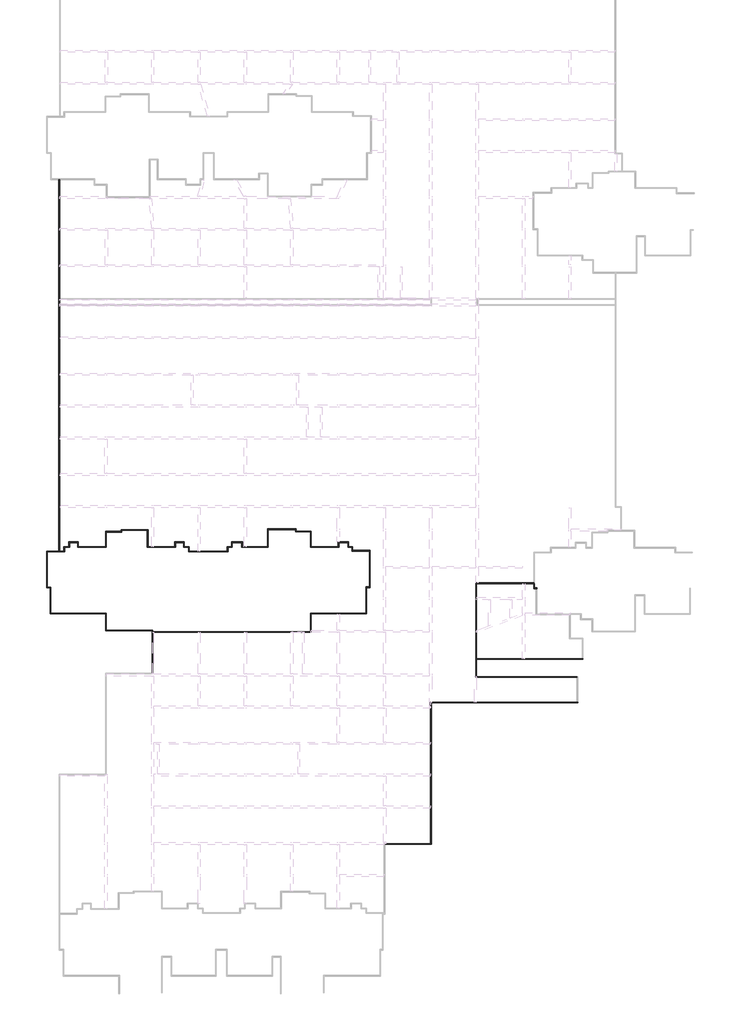
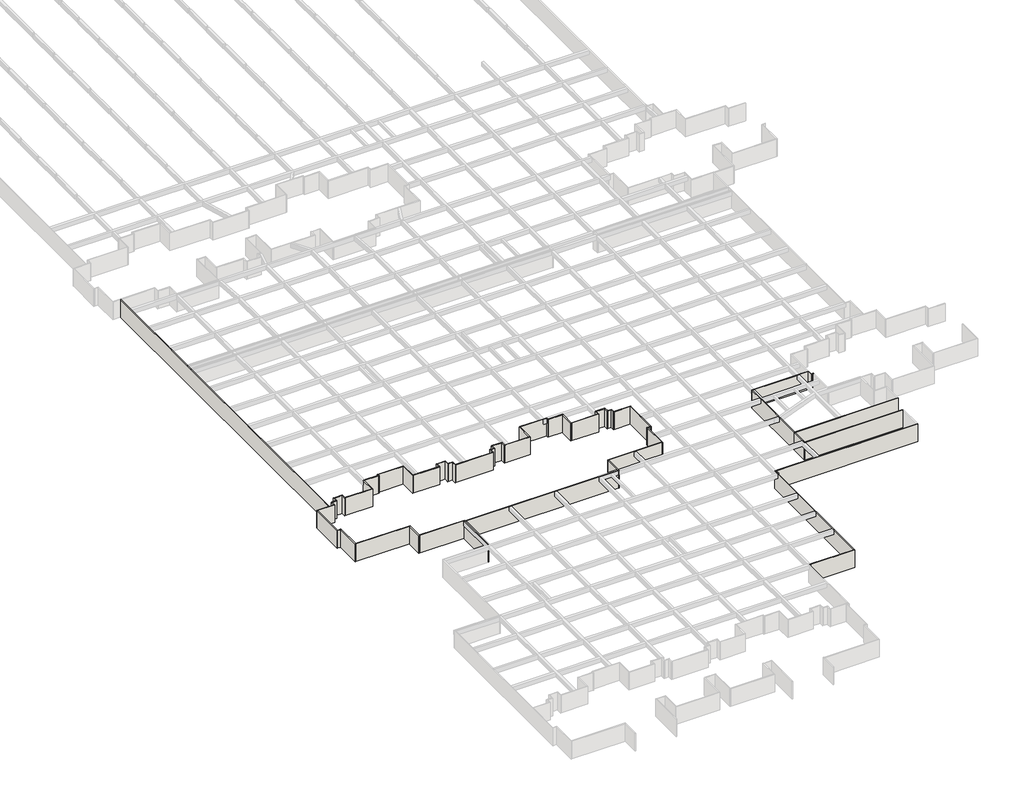
# One storey, part 2 of 14: 61 walls.
"""IFC4 building model written with IfcOpenShell, lengths in millimetres."""

from ifc_helpers import new_model, si_unit, origin, origin_with_axes, place, context, project, spatial, polyline, outline, extrude, faceted_brep, element, save

model = new_model("IFC4")

# Units and contexts
model_context = context("Model", 3, world=origin())
ifc_project = project(units=[si_unit("LENGTHUNIT", "METRE", prefix="MILLI")], contexts=[model_context])

# Site, building, storey
site = spatial("IfcSite", under=ifc_project)
building = spatial("IfcBuilding", under=site)
storey = spatial("IfcBuildingStorey", under=building, Name="户型图", Elevation=0.0)

# Walls
placement = place(None, origin())
element("IfcWall", 1, ObjectType="所有墙体", at=placement, inside=storey, context=model_context, shape_type="Brep", body=[
    faceted_brep([(-594257.5937933, -107575.8355437, 0.0), (-594257.5937933, -171682.856538, 0.0), (-594257.5937933, -171682.856538, 3300.0), (-594257.5937933, -107575.8355437, 3300.0), (-594137.5937933, -107575.8355437, 0.0), (-594137.5937933, -107575.8355437, 3300.0), (-594137.5937933, -128099.4327532, 3300.0), (-594137.5937933, -128219.4327532, 3300.0), (-594137.5937933, -129174.4327531, 3300.0), (-594137.5937933, -129294.4327531, 3300.0), (-594137.5937933, -171682.856538, 3300.0), (-594137.5937933, -171682.856538, 0.0), (-594137.5937933, -129294.4327531, 0.0), (-594137.5937933, -129174.4327531, 0.0), (-594137.5937933, -128219.4327532, 0.0), (-594137.5937933, -128099.4327532, 0.0)], [[[0, 1, 2, 3]], [[4, 5, 6, 7, 8, 9, 10, 11, 12, 13, 14, 15]], [[1, 0, 4, 15, 14, 13, 12, 11]], [[3, 2, 10, 9, 8, 7, 6, 5]], [[0, 3, 5, 4]], [[2, 1, 11, 10]]]),
])
element("IfcWall", 2, ObjectType="所有墙体", at=placement, inside=storey, context=model_context, shape_type="Brep", body=[
    faceted_brep([(-593271.2602583, -171682.856538, 0.0), (-593391.2602583, -171682.856538, 0.0), (-594137.5937933, -171682.856538, 0.0), (-594257.5937933, -171682.856538, 0.0), (-596391.260259, -171682.856538, 0.0), (-596391.260259, -171682.856538, 3300.0), (-594257.5937933, -171682.856538, 3300.0), (-594137.5937933, -171682.856538, 3300.0), (-593391.2602583, -171682.856538, 3300.0), (-593271.2602583, -171682.856538, 3300.0), (-593271.2602583, -171802.856538, 0.0), (-593271.2602583, -171802.856538, 3300.0), (-596271.260259, -171802.856538, 3300.0), (-596391.260259, -171802.856538, 3300.0), (-596391.260259, -171802.856538, 0.0), (-596271.260259, -171802.856538, 0.0)], [[[0, 1, 2, 3, 4, 5, 6, 7, 8, 9]], [[10, 11, 12, 13, 14, 15]], [[4, 3, 2, 1, 0, 10, 15, 14]], [[9, 8, 7, 6, 5, 13, 12, 11]], [[5, 4, 14, 13]], [[0, 9, 11, 10]]]),
])
element("IfcWall", 3, ObjectType="所有墙体", at=placement, inside=storey, context=model_context, shape_type="Brep", body=[
    faceted_brep([(-596391.260259, -171802.856538, 0.0), (-596391.260259, -178002.8565379, 0.0), (-596391.260259, -178002.8565379, 3300.0), (-596391.260259, -171802.856538, 3300.0), (-596271.260259, -171802.856538, 0.0), (-596271.260259, -171802.856538, 3300.0), (-596271.260259, -177882.8565379, 3300.0), (-596271.260259, -178002.8565379, 3300.0), (-596271.260259, -178002.8565379, 0.0), (-596271.260259, -177882.8565379, 0.0)], [[[0, 1, 2, 3]], [[4, 5, 6, 7, 8, 9]], [[1, 0, 4, 9, 8]], [[3, 2, 7, 6, 5]], [[0, 3, 5, 4]], [[2, 1, 8, 7]]]),
])
element("IfcWall", 4, ObjectType="所有墙体", at=placement, inside=storey, context=model_context, shape_type="Brep", body=[
    faceted_brep([(-596271.260259, -178002.8565379, 0.0), (-595791.2602578, -178002.8565379, 0.0), (-595671.2602578, -178002.8565379, 0.0), (-595671.2602578, -178002.8565379, 3300.0), (-595791.2602578, -178002.8565379, 3300.0), (-596271.260259, -178002.8565379, 3300.0), (-596271.260259, -177882.8565379, 0.0), (-596271.260259, -177882.8565379, 3300.0), (-595671.2602578, -177882.8565379, 3300.0), (-595671.2602578, -177882.8565379, 0.0)], [[[0, 1, 2, 3, 4, 5]], [[6, 7, 8, 9]], [[2, 1, 0, 6, 9]], [[5, 4, 3, 8, 7]], [[0, 5, 7, 6]], [[3, 2, 9, 8]]]),
])
element("IfcWall", 5, ObjectType="所有墙体", at=placement, inside=storey, context=model_context, shape_type="Brep", body=[
    faceted_brep([(-595791.2602578, -178002.8565379, 0.0), (-595791.2602578, -182502.856538, 0.0), (-595791.2602578, -182502.856538, 3300.0), (-595791.2602578, -178002.8565379, 3300.0), (-595671.2602578, -178002.8565379, 0.0), (-595671.2602578, -178002.8565379, 3300.0), (-595671.2602578, -182382.856538, 3300.0), (-595671.2602578, -182502.856538, 3300.0), (-595671.2602578, -182502.856538, 0.0), (-595671.2602578, -182382.856538, 0.0)], [[[0, 1, 2, 3]], [[4, 5, 6, 7, 8, 9]], [[1, 0, 4, 9, 8]], [[3, 2, 7, 6, 5]], [[0, 3, 5, 4]], [[2, 1, 8, 7]]]),
])
element("IfcWall", 6, ObjectType="所有墙体", at=placement, inside=storey, context=model_context, shape_type="Brep", body=[
    faceted_brep([(-595671.2602578, -182502.856538, 0.0), (-586191.2602569, -182502.856538, 0.0), (-586071.2602569, -182502.856538, 0.0), (-586071.2602569, -182502.856538, 3300.0), (-586191.2602569, -182502.856538, 3300.0), (-595671.2602578, -182502.856538, 3300.0), (-595671.2602578, -182382.856538, 0.0), (-595671.2602578, -182382.856538, 3300.0), (-586071.2602569, -182382.856538, 3300.0), (-586071.2602569, -182382.856538, 0.0)], [[[0, 1, 2, 3, 4, 5]], [[6, 7, 8, 9]], [[2, 1, 0, 6, 9]], [[5, 4, 3, 8, 7]], [[0, 5, 7, 6]], [[3, 2, 9, 8]]]),
])
element("IfcWall", 7, ObjectType="所有墙体", at=placement, inside=storey, context=model_context, shape_type="Brep", body=[
    faceted_brep([(-586191.2602569, -182502.856538, 0.0), (-586191.2602569, -185431.2417661, 0.0), (-586191.2602569, -185431.2417661, 3300.0), (-586191.2602569, -182502.856538, 3300.0), (-586071.2602569, -182502.856538, 0.0), (-586071.2602569, -182502.856538, 3300.0), (-586071.2602569, -185311.2417661, 3300.0), (-586071.2602569, -185431.2417661, 3300.0), (-586071.2602569, -185431.2417661, 0.0), (-586071.2602569, -185311.2417661, 0.0)], [[[0, 1, 2, 3]], [[4, 5, 6, 7, 8, 9]], [[1, 0, 4, 9, 8]], [[3, 2, 7, 6, 5]], [[0, 3, 5, 4]], [[2, 1, 8, 7]]]),
])
element("IfcWall", 8, ObjectType="所有墙体", at=placement, inside=storey, context=model_context, shape_type="Brep", body=[
    faceted_brep([(-586071.2602569, -185431.2417661, 0.0), (-578191.2602569, -185431.2417661, 0.0), (-578071.2602569, -185431.2417661, 0.0), (-578071.2602569, -185431.2417661, 3300.0), (-578191.2602569, -185431.2417661, 3300.0), (-578267.6529954, -185431.2417661, 3300.0), (-586071.2602569, -185431.2417661, 3300.0), (-586071.2602569, -185311.2417661, 0.0), (-586071.2602569, -185311.2417661, 3300.0), (-578071.2602569, -185311.2417661, 3300.0), (-578071.2602569, -185311.2417661, 0.0), (-578071.2602569, -185371.5491398, 3300.0)], [[[0, 1, 2, 3, 4, 5, 6]], [[7, 8, 9, 10]], [[2, 1, 0, 7, 10]], [[6, 5, 4, 3, 11, 9, 8]], [[0, 6, 8, 7]], [[3, 2, 10, 9, 11]]]),
])
element("IfcWall", 9, ObjectType="所有墙体", at=placement, inside=storey, context=model_context, shape_type="Brep", body=[
    faceted_brep([(-578191.2602569, -185431.2417661, 0.0), (-578191.2602569, -192711.2417661, 0.0), (-578191.2602569, -192831.2417661, 0.0), (-578191.2602569, -192831.2417661, 3300.0), (-578191.2602569, -192711.2417661, 3300.0), (-578191.2602569, -185431.2417661, 3300.0), (-578191.2602569, -185431.2417661, 2500.0), (-578071.2602569, -185431.2417661, 0.0), (-578071.2602569, -185431.2417661, 3300.0), (-578071.2602569, -185532.8564588, 3300.0), (-578071.2602569, -185652.8564588, 3300.0), (-578071.2602569, -192831.2417661, 3300.0), (-578071.2602569, -192831.2417661, 2500.0), (-578071.2602569, -192831.2417661, 0.0), (-578071.2602569, -185652.8564588, 0.0), (-578071.2602569, -185532.8564588, 0.0)], [[[0, 1, 2, 3, 4, 5, 6]], [[7, 8, 9, 10, 11, 12, 13, 14, 15]], [[2, 1, 0, 7, 15, 14, 13]], [[5, 4, 3, 11, 10, 9, 8]], [[0, 6, 5, 8, 7]], [[3, 2, 13, 12, 11]]]),
])
element("IfcWall", 10, ObjectType="所有墙体", at=placement, inside=storey, context=model_context, shape_type="Brep", body=[
    faceted_brep([(-537997.7352575, -222250.9174567, 0.0), (-529997.7352575, -222250.9174567, 0.0), (-529997.7352575, -222250.9174567, 3300.0), (-537831.2602569, -222250.9174567, 3300.0), (-537997.7352575, -222250.9174567, 3300.0), (-537997.7352575, -222250.9174567, 2500.0), (-537997.7352575, -222130.9174567, 0.0), (-537997.7352575, -222130.9174567, 3300.0), (-537831.2602569, -222130.9174567, 3300.0), (-530117.7352575, -222130.9174567, 3300.0), (-529997.7352575, -222130.9174567, 3300.0), (-529997.7352575, -222130.9174567, 0.0), (-530117.7352575, -222130.9174567, 0.0)], [[[0, 1, 2, 3, 4, 5]], [[6, 7, 8, 9, 10, 11, 12]], [[1, 0, 6, 12, 11]], [[4, 3, 2, 10, 9, 8, 7]], [[0, 5, 4, 7, 6]], [[2, 1, 11, 10]]]),
])
element("IfcWall", 11, ObjectType="所有墙体", at=placement, inside=storey, context=model_context, shape_type="Brep", body=[
    faceted_brep([(-529997.7352575, -222130.9174567, 0.0), (-529997.7352575, -197850.9174567, 0.0), (-529997.7352575, -197730.9174567, 0.0), (-529997.7352575, -197730.9174567, 3300.0), (-529997.7352575, -197850.9174567, 3300.0), (-529997.7352575, -198534.4327531, 3300.0), (-529997.7352575, -222130.9174567, 3300.0), (-530117.7352575, -222130.9174567, 0.0), (-530117.7352575, -222130.9174567, 3300.0), (-530117.7352575, -198534.4327531, 3300.0), (-530117.7352575, -197730.9174567, 3300.0), (-530117.7352575, -197730.9174567, 2500.0), (-530117.7352575, -197730.9174567, 0.0)], [[[0, 1, 2, 3, 4, 5, 6]], [[7, 8, 9, 10, 11, 12]], [[2, 1, 0, 7, 12]], [[6, 5, 4, 3, 10, 9, 8]], [[0, 6, 8, 7]], [[3, 2, 12, 11, 10]]]),
])
element("IfcWall", 12, ObjectType="所有墙体", at=placement, inside=storey, context=model_context, shape_type="Brep", body=[
    faceted_brep([(-529997.7352575, -197850.9174567, 0.0), (-504707.6529953, -197850.9174567, 0.0), (-504707.6529953, -197850.9174567, 3300.0), (-529867.6529954, -197850.9174567, 3300.0), (-529997.7352575, -197850.9174567, 3300.0), (-529997.7352575, -197850.9174567, 2500.0), (-529997.7352575, -197730.9174567, 0.0), (-529997.7352575, -197730.9174567, 3300.0), (-529867.6529954, -197730.9174567, 3300.0), (-504827.6529953, -197730.9174567, 3300.0), (-504707.6529953, -197730.9174567, 3300.0), (-504707.6529953, -197730.9174567, 0.0), (-504827.6529953, -197730.9174567, 0.0)], [[[0, 1, 2, 3, 4, 5]], [[6, 7, 8, 9, 10, 11, 12]], [[1, 0, 6, 12, 11]], [[4, 3, 2, 10, 9, 8, 7]], [[0, 5, 4, 7, 6]], [[2, 1, 11, 10]]]),
])
element("IfcWall", 13, ObjectType="所有墙体", at=placement, inside=storey, context=model_context, shape_type="Brep", body=[
    faceted_brep([(-504827.6529953, -193330.9174567, 0.0), (-522195.6671501, -193330.9174567, 0.0), (-522315.6671501, -193330.9174567, 0.0), (-522315.6671501, -193330.9174567, 3300.0), (-522195.6671501, -193330.9174567, 3300.0), (-522167.6529953, -193330.9174567, 3300.0), (-504827.6529953, -193330.9174567, 3300.0), (-504827.6529953, -193450.9174567, 0.0), (-504827.6529953, -193450.9174567, 3300.0), (-522167.6529953, -193450.9174567, 3300.0), (-522315.6671501, -193450.9174567, 3300.0), (-522315.6671501, -193450.9174567, 2500.0), (-522315.6671501, -193450.9174567, 0.0)], [[[0, 1, 2, 3, 4, 5, 6]], [[7, 8, 9, 10, 11, 12]], [[2, 1, 0, 7, 12]], [[6, 5, 4, 3, 10, 9, 8]], [[0, 6, 8, 7]], [[3, 2, 12, 11, 10]]]),
])
element("IfcWall", 14, ObjectType="所有墙体", at=placement, inside=storey, context=model_context, shape_type="Brep", body=[
    faceted_brep([(-522195.6671501, -193330.9174567, 0.0), (-522195.6671501, -190350.9174567, 0.0), (-522195.6671501, -190230.9174567, 0.0), (-522195.6671501, -190230.9174567, 3300.0), (-522195.6671501, -190350.9174567, 3300.0), (-522195.6671501, -192842.8565135, 3300.0), (-522195.6671501, -193330.9174567, 3300.0), (-522195.6671501, -193330.9174567, 2500.0), (-522315.6671501, -193330.9174567, 0.0), (-522315.6671501, -193330.9174567, 3300.0), (-522315.6671501, -193242.8565135, 3300.0), (-522315.6671501, -190230.9174567, 3300.0), (-522315.6671501, -190230.9174567, 0.0), (-522303.9222774, -190230.9174567, 0.0), (-522303.9222774, -190230.9174567, 3300.0)], [[[0, 1, 2, 3, 4, 5, 6, 7]], [[8, 9, 10, 11, 12]], [[2, 1, 0, 8, 12, 13]], [[6, 5, 4, 3, 14, 11, 10, 9]], [[0, 7, 6, 9, 8]], [[3, 2, 13, 12, 11, 14]]]),
])
element("IfcWall", 15, ObjectType="所有墙体", at=placement, inside=storey, context=model_context, shape_type="Brep", body=[
    faceted_brep([(-522195.6671501, -190350.9174567, 0.0), (-503834.8997281, -190350.9174567, 0.0), (-503834.8997281, -190350.9174567, 3300.0), (-522195.6671501, -190350.9174567, 3300.0), (-522195.6671501, -190230.9174567, 0.0), (-522195.6671501, -190230.9174567, 3300.0), (-522183.9222774, -190230.9174567, 3300.0), (-503954.8997281, -190230.9174567, 3300.0), (-503834.8997281, -190230.9174567, 3300.0), (-503834.8997281, -190230.9174567, 0.0), (-503954.8997281, -190230.9174567, 0.0), (-522183.9222774, -190230.9174567, 0.0)], [[[0, 1, 2, 3]], [[4, 5, 6, 7, 8, 9, 10, 11]], [[1, 0, 4, 11, 10, 9]], [[3, 2, 8, 7, 6, 5]], [[0, 3, 5, 4]], [[2, 1, 9, 8]]]),
])
element("IfcWall", 16, ObjectType="所有墙体", at=placement, inside=storey, context=model_context, shape_type="Brep", body=[
    faceted_brep([(-512303.9222774, -177127.2416788, 0.0), (-522303.9222774, -177127.2416788, 0.0), (-522303.9222774, -177127.2416788, 3300.0), (-514267.6529954, -177127.2416788, 3300.0), (-513867.6529954, -177127.2416788, 3300.0), (-512303.9222774, -177127.2416788, 3300.0), (-512303.9222774, -177247.2416788, 0.0), (-512303.9222774, -177247.2416788, 3300.0), (-513867.6529954, -177247.2416788, 3300.0), (-514267.6529954, -177247.2416788, 3300.0), (-522183.9222774, -177247.2416788, 3300.0), (-522303.9222774, -177247.2416788, 3300.0), (-522303.9222774, -177247.2416788, 0.0), (-522183.9222774, -177247.2416788, 0.0)], [[[0, 1, 2, 3, 4, 5]], [[6, 7, 8, 9, 10, 11, 12, 13]], [[1, 0, 6, 13, 12]], [[5, 4, 3, 2, 11, 10, 9, 8, 7]], [[0, 5, 7, 6]], [[2, 1, 12, 11]]]),
])
element("IfcWall", 17, ObjectType="所有墙体", at=placement, inside=storey, context=model_context, shape_type="Brep", body=[
    faceted_brep([(-522303.9222774, -177247.2416788, 0.0), (-522303.9222774, -190230.9174567, 0.0), (-522303.9222774, -190230.9174567, 3300.0), (-522303.9222774, -185692.8565135, 3300.0), (-522303.9222774, -185367.2051019, 3300.0), (-522303.9222774, -185292.8565135, 3300.0), (-522303.9222774, -180052.8565433, 3300.0), (-522303.9222774, -179652.8565433, 3300.0), (-522303.9222774, -177247.2416788, 3300.0), (-522183.9222774, -177247.2416788, 0.0), (-522183.9222774, -177247.2416788, 2500.0), (-522183.9222774, -177247.2416788, 3300.0), (-522183.9222774, -179652.8565433, 3300.0), (-522183.9222774, -180052.8565433, 3300.0), (-522183.9222774, -185292.8565135, 3300.0), (-522183.9222774, -185322.6756033, 3300.0), (-522183.9222774, -185692.8565135, 3300.0), (-522183.9222774, -190230.9174567, 3300.0), (-522183.9222774, -190230.9174567, 0.0), (-522195.6671501, -190230.9174567, 0.0), (-522195.6671501, -190230.9174567, 3300.0)], [[[0, 1, 2, 3, 4, 5, 6, 7, 8]], [[9, 10, 11, 12, 13, 14, 15, 16, 17, 18]], [[1, 0, 9, 18, 19]], [[8, 7, 6, 5, 4, 3, 2, 20, 17, 16, 15, 14, 13, 12, 11]], [[0, 8, 11, 10, 9]], [[2, 1, 19, 18, 17, 20]]]),
])
element("IfcWall", 18, ObjectType="所有墙体", at=placement, inside=storey, context=model_context, shape_type="Brep", body=[
    faceted_brep([(-593271.2602583, -171682.856538, 0.0), (-593271.2602583, -171002.8565379, 0.0), (-593271.2602583, -170882.8565379, 0.0), (-593271.2602583, -170882.8565379, 3300.0), (-593271.2602583, -171002.8565379, 3300.0), (-593271.2602583, -171682.856538, 3300.0), (-593391.2602583, -171682.856538, 0.0), (-593391.2602583, -171682.856538, 3300.0), (-593391.2602583, -170882.8565379, 3300.0), (-593391.2602583, -170882.8565379, 0.0)], [[[0, 1, 2, 3, 4, 5]], [[6, 7, 8, 9]], [[2, 1, 0, 6, 9]], [[5, 4, 3, 8, 7]], [[0, 5, 7, 6]], [[3, 2, 9, 8]]]),
])
element("IfcWall", 19, ObjectType="所有墙体", at=placement, inside=storey, context=model_context, shape_type="Brep", body=[
    faceted_brep([(-593271.2602583, -171002.8565379, 0.0), (-592421.2602592, -171002.8565379, 0.0), (-592421.2602592, -171002.8565379, 3300.0), (-593271.2602583, -171002.8565379, 3300.0), (-593271.2602583, -170882.8565379, 0.0), (-593271.2602583, -170882.8565379, 3300.0), (-592541.2602592, -170882.8565379, 3300.0), (-592421.2602592, -170882.8565379, 3300.0), (-592421.2602592, -170882.8565379, 0.0), (-592541.2602592, -170882.8565379, 0.0)], [[[0, 1, 2, 3]], [[4, 5, 6, 7, 8, 9]], [[1, 0, 4, 9, 8]], [[3, 2, 7, 6, 5]], [[0, 3, 5, 4]], [[2, 1, 8, 7]]]),
])
element("IfcWall", 20, ObjectType="所有墙体", at=placement, inside=storey, context=model_context, shape_type="Brep", body=[
    faceted_brep([(-592421.2602592, -170882.8565379, 0.0), (-592421.2602592, -170202.8565379, 0.0), (-592421.2602592, -170082.8565379, 0.0), (-592421.2602592, -170082.8565379, 3300.0), (-592421.2602592, -170202.8565379, 3300.0), (-592421.2602592, -170882.8565379, 3300.0), (-592541.2602592, -170882.8565379, 0.0), (-592541.2602592, -170882.8565379, 3300.0), (-592541.2602592, -170082.8565379, 3300.0), (-592541.2602592, -170082.8565379, 0.0)], [[[0, 1, 2, 3, 4, 5]], [[6, 7, 8, 9]], [[2, 1, 0, 6, 9]], [[5, 4, 3, 8, 7]], [[0, 5, 7, 6]], [[3, 2, 9, 8]]]),
])
element("IfcWall", 21, ObjectType="所有墙体", at=placement, inside=storey, context=model_context, shape_type="Brep", body=[
    faceted_brep([(-592421.2602592, -170202.8565379, 0.0), (-591041.2602596, -170202.8565379, 0.0), (-590921.2602596, -170202.8565379, 0.0), (-590921.2602596, -170202.8565379, 3300.0), (-591041.2602596, -170202.8565379, 3300.0), (-592421.2602592, -170202.8565379, 3300.0), (-592421.2602592, -170082.8565379, 0.0), (-592421.2602592, -170082.8565379, 3300.0), (-590921.2602596, -170082.8565379, 3300.0), (-590921.2602596, -170082.8565379, 0.0)], [[[0, 1, 2, 3, 4, 5]], [[6, 7, 8, 9]], [[2, 1, 0, 6, 9]], [[5, 4, 3, 8, 7]], [[0, 5, 7, 6]], [[3, 2, 9, 8]]]),
])
element("IfcWall", 22, ObjectType="所有墙体", at=placement, inside=storey, context=model_context, shape_type="Brep", body=[
    faceted_brep([(-591041.2602596, -170202.8565379, 0.0), (-591041.2602596, -171002.8565379, 0.0), (-591041.2602596, -171002.8565379, 3300.0), (-591041.2602596, -170202.8565379, 3300.0), (-590921.2602596, -170202.8565379, 0.0), (-590921.2602596, -170202.8565379, 3300.0), (-590921.2602596, -170882.8565379, 3300.0), (-590921.2602596, -171002.8565379, 3300.0), (-590921.2602596, -171002.8565379, 0.0), (-590921.2602596, -170882.8565379, 0.0)], [[[0, 1, 2, 3]], [[4, 5, 6, 7, 8, 9]], [[1, 0, 4, 9, 8]], [[3, 2, 7, 6, 5]], [[0, 3, 5, 4]], [[2, 1, 8, 7]]]),
])
element("IfcWall", 23, ObjectType="所有墙体", at=placement, inside=storey, context=model_context, shape_type="Brep", body=[
    faceted_brep([(-590921.2602596, -171002.8565379, 0.0), (-586071.2602569, -171002.8565379, 0.0), (-586071.2602569, -171002.8565379, 3300.0), (-590921.2602596, -171002.8565379, 3300.0), (-590921.2602596, -170882.8565379, 0.0), (-590921.2602596, -170882.8565379, 3300.0), (-586191.2602569, -170882.8565379, 3300.0), (-586071.2602569, -170882.8565379, 3300.0), (-586071.2602569, -170882.8565379, 0.0), (-586191.2602569, -170882.8565379, 0.0)], [[[0, 1, 2, 3]], [[4, 5, 6, 7, 8, 9]], [[1, 0, 4, 9, 8]], [[3, 2, 7, 6, 5]], [[0, 3, 5, 4]], [[2, 1, 8, 7]]]),
])
element("IfcWall", 24, ObjectType="所有墙体", at=placement, inside=storey, context=model_context, shape_type="Brep", body=[
    faceted_brep([(-586071.2602569, -170882.8565379, 0.0), (-586071.2602569, -168377.8565288, 0.0), (-586071.2602569, -168257.8565288, 0.0), (-586071.2602569, -168257.8565288, 3300.0), (-586071.2602569, -168377.8565288, 3300.0), (-586071.2602569, -170882.8565379, 3300.0), (-586191.2602569, -170882.8565379, 0.0), (-586191.2602569, -170882.8565379, 3300.0), (-586191.2602569, -168377.8565288, 3300.0), (-586191.2602569, -168257.8565288, 3300.0), (-586191.2602569, -168257.8565288, 2500.0), (-586191.2602569, -168257.8565288, 0.0)], [[[0, 1, 2, 3, 4, 5]], [[6, 7, 8, 9, 10, 11]], [[2, 1, 0, 6, 11]], [[5, 4, 3, 9, 8, 7]], [[0, 5, 7, 6]], [[3, 2, 11, 10, 9]]]),
])
element("IfcWall", 25, ObjectType="所有墙体", at=placement, inside=storey, context=model_context, shape_type="SweptSolid", body=[
    extrude(outline(polyline([(-583541.2602598, -168377.8565288), (-586071.2602569, -168377.8565288), (-586071.2602569, -168257.8565288), (-583541.2602598, -168257.8565288), (-583541.2602598, -168377.8565288)])), origin_with_axes(), (0.0, 0.0, 1.0), 3300.0),
])
element("IfcWall", 26, ObjectType="所有墙体", at=placement, inside=storey, context=model_context, shape_type="Brep", body=[
    faceted_brep([(-583421.2602598, -168377.8565288, 0.0), (-583421.2602598, -168102.8565288, 0.0), (-583421.2602598, -167982.8565288, 0.0), (-583421.2602598, -167982.8565288, 3300.0), (-583421.2602598, -168102.8565288, 3300.0), (-583421.2602598, -168377.8565288, 3300.0), (-583541.2602598, -168377.8565288, 0.0), (-583541.2602598, -168377.8565288, 3300.0), (-583541.2602598, -168257.8565288, 3300.0), (-583541.2602598, -167982.8565288, 3300.0), (-583541.2602598, -167982.8565288, 0.0), (-583541.2602598, -168257.8565288, 0.0)], [[[0, 1, 2, 3, 4, 5]], [[6, 7, 8, 9, 10, 11]], [[2, 1, 0, 6, 11, 10]], [[5, 4, 3, 9, 8, 7]], [[0, 5, 7, 6]], [[3, 2, 10, 9]]]),
])
element("IfcWall", 27, ObjectType="所有墙体", at=placement, inside=storey, context=model_context, shape_type="Brep", body=[
    faceted_brep([(-583421.2602598, -168102.8565288, 0.0), (-578991.2602535, -168102.8565288, 0.0), (-578871.2602535, -168102.8565288, 0.0), (-578871.2602535, -168102.8565288, 3300.0), (-578991.2602535, -168102.8565288, 3300.0), (-583421.2602598, -168102.8565288, 3300.0), (-583421.2602598, -167982.8565288, 0.0), (-583421.2602598, -167982.8565288, 3300.0), (-578871.2602535, -167982.8565288, 3300.0), (-578871.2602535, -167982.8565288, 0.0)], [[[0, 1, 2, 3, 4, 5]], [[6, 7, 8, 9]], [[2, 1, 0, 6, 9]], [[5, 4, 3, 8, 7]], [[0, 5, 7, 6]], [[3, 2, 9, 8]]]),
])
element("IfcWall", 28, ObjectType="所有墙体", at=placement, inside=storey, context=model_context, shape_type="Brep", body=[
    faceted_brep([(-578991.2602535, -168102.8565288, 0.0), (-578991.2602535, -171002.8565379, 0.0), (-578991.2602535, -171002.8565379, 3300.0), (-578991.2602535, -168102.8565288, 3300.0), (-578871.2602535, -168102.8565288, 0.0), (-578871.2602535, -168102.8565288, 3300.0), (-578871.2602535, -170882.8565379, 3300.0), (-578871.2602535, -171002.8565379, 3300.0), (-578871.2602535, -171002.8565379, 0.0), (-578871.2602535, -170882.8565379, 0.0)], [[[0, 1, 2, 3]], [[4, 5, 6, 7, 8, 9]], [[1, 0, 4, 9, 8]], [[3, 2, 7, 6, 5]], [[0, 3, 5, 4]], [[2, 1, 8, 7]]]),
])
element("IfcWall", 29, ObjectType="所有墙体", at=placement, inside=storey, context=model_context, shape_type="Brep", body=[
    faceted_brep([(-578871.2602535, -171002.8565379, 0.0), (-574121.2602591, -171002.8565379, 0.0), (-574121.2602591, -171002.8565379, 3300.0), (-578871.2602535, -171002.8565379, 3300.0), (-578871.2602535, -170882.8565379, 0.0), (-578871.2602535, -170882.8565379, 3300.0), (-574241.2602591, -170882.8565379, 3300.0), (-574121.2602591, -170882.8565379, 3300.0), (-574121.2602591, -170882.8565379, 0.0), (-574241.2602591, -170882.8565379, 0.0)], [[[0, 1, 2, 3]], [[4, 5, 6, 7, 8, 9]], [[1, 0, 4, 9, 8]], [[3, 2, 7, 6, 5]], [[0, 3, 5, 4]], [[2, 1, 8, 7]]]),
])
element("IfcWall", 30, ObjectType="所有墙体", at=placement, inside=storey, context=model_context, shape_type="Brep", body=[
    faceted_brep([(-574121.2602591, -170882.8565379, 0.0), (-574121.2602591, -170202.8565379, 0.0), (-574121.2602591, -170082.8565379, 0.0), (-574121.2602591, -170082.8565379, 3300.0), (-574121.2602591, -170202.8565379, 3300.0), (-574121.2602591, -170882.8565379, 3300.0), (-574241.2602591, -170882.8565379, 0.0), (-574241.2602591, -170882.8565379, 3300.0), (-574241.2602591, -170082.8565379, 3300.0), (-574241.2602591, -170082.8565379, 0.0)], [[[0, 1, 2, 3, 4, 5]], [[6, 7, 8, 9]], [[2, 1, 0, 6, 9]], [[5, 4, 3, 8, 7]], [[0, 5, 7, 6]], [[3, 2, 9, 8]]]),
])
element("IfcWall", 31, ObjectType="所有墙体", at=placement, inside=storey, context=model_context, shape_type="Brep", body=[
    faceted_brep([(-574121.2602591, -170202.8565379, 0.0), (-572741.2602596, -170202.8565379, 0.0), (-572621.2602596, -170202.8565379, 0.0), (-572621.2602596, -170202.8565379, 3300.0), (-572741.2602596, -170202.8565379, 3300.0), (-574121.2602591, -170202.8565379, 3300.0), (-574121.2602591, -170082.8565379, 0.0), (-574121.2602591, -170082.8565379, 3300.0), (-572621.2602596, -170082.8565379, 3300.0), (-572621.2602596, -170082.8565379, 0.0)], [[[0, 1, 2, 3, 4, 5]], [[6, 7, 8, 9]], [[2, 1, 0, 6, 9]], [[5, 4, 3, 8, 7]], [[0, 5, 7, 6]], [[3, 2, 9, 8]]]),
])
element("IfcWall", 32, ObjectType="所有墙体", at=placement, inside=storey, context=model_context, shape_type="Brep", body=[
    faceted_brep([(-572741.2602596, -170202.8565379, 0.0), (-572741.2602596, -171002.8565379, 0.0), (-572741.2602596, -171002.8565379, 3300.0), (-572741.2602596, -170202.8565379, 3300.0), (-572621.2602596, -170202.8565379, 0.0), (-572621.2602596, -170202.8565379, 3300.0), (-572621.2602596, -170882.8565379, 3300.0), (-572621.2602596, -171002.8565379, 3300.0), (-572621.2602596, -171002.8565379, 0.0), (-572621.2602596, -170882.8565379, 0.0)], [[[0, 1, 2, 3]], [[4, 5, 6, 7, 8, 9]], [[1, 0, 4, 9, 8]], [[3, 2, 7, 6, 5]], [[0, 3, 5, 4]], [[2, 1, 8, 7]]]),
])
element("IfcWall", 33, ObjectType="所有墙体", at=placement, inside=storey, context=model_context, shape_type="Brep", body=[
    faceted_brep([(-572621.2602596, -171002.8565379, 0.0), (-571891.2602524, -171002.8565379, 0.0), (-571771.2602524, -171002.8565379, 0.0), (-571771.2602524, -171002.8565379, 3300.0), (-571891.2602524, -171002.8565379, 3300.0), (-572621.2602596, -171002.8565379, 3300.0), (-572621.2602596, -170882.8565379, 0.0), (-572621.2602596, -170882.8565379, 3300.0), (-571771.2602524, -170882.8565379, 3300.0), (-571771.2602524, -170882.8565379, 0.0)], [[[0, 1, 2, 3, 4, 5]], [[6, 7, 8, 9]], [[2, 1, 0, 6, 9]], [[5, 4, 3, 8, 7]], [[0, 5, 7, 6]], [[3, 2, 9, 8]]]),
])
element("IfcWall", 34, ObjectType="所有墙体", at=placement, inside=storey, context=model_context, shape_type="Brep", body=[
    faceted_brep([(-571891.2602524, -171002.8565379, 0.0), (-571891.2602524, -171802.856538, 0.0), (-571891.2602524, -171802.856538, 3300.0), (-571891.2602524, -171002.8565379, 3300.0), (-571771.2602524, -171002.8565379, 0.0), (-571771.2602524, -171002.8565379, 3300.0), (-571771.2602524, -171682.856538, 3300.0), (-571771.2602524, -171802.856538, 3300.0), (-571771.2602524, -171802.856538, 0.0), (-571771.2602524, -171682.856538, 0.0)], [[[0, 1, 2, 3]], [[4, 5, 6, 7, 8, 9]], [[1, 0, 4, 9, 8]], [[3, 2, 7, 6, 5]], [[0, 3, 5, 4]], [[2, 1, 8, 7]]]),
])
element("IfcWall", 35, ObjectType="所有墙体", at=placement, inside=storey, context=model_context, shape_type="Brep", body=[
    faceted_brep([(-571771.2602524, -171802.856538, 0.0), (-565071.2602567, -171802.856538, 0.0), (-565071.2602567, -171802.856538, 3300.0), (-571771.2602524, -171802.856538, 3300.0), (-571771.2602524, -171682.856538, 0.0), (-571771.2602524, -171682.856538, 3300.0), (-565191.2602567, -171682.856538, 3300.0), (-565071.2602567, -171682.856538, 3300.0), (-565071.2602567, -171682.856538, 0.0), (-565191.2602567, -171682.856538, 0.0)], [[[0, 1, 2, 3]], [[4, 5, 6, 7, 8, 9]], [[1, 0, 4, 9, 8]], [[3, 2, 7, 6, 5]], [[0, 3, 5, 4]], [[2, 1, 8, 7]]]),
])
element("IfcWall", 36, ObjectType="所有墙体", at=placement, inside=storey, context=model_context, shape_type="Brep", body=[
    faceted_brep([(-565071.2602567, -171682.856538, 0.0), (-565071.2602567, -171002.8565379, 0.0), (-565071.2602567, -170882.8565379, 0.0), (-565071.2602567, -170882.8565379, 3300.0), (-565071.2602567, -171002.8565379, 3300.0), (-565071.2602567, -171682.856538, 3300.0), (-565191.2602567, -171682.856538, 0.0), (-565191.2602567, -171682.856538, 3300.0), (-565191.2602567, -170882.8565379, 3300.0), (-565191.2602567, -170882.8565379, 0.0)], [[[0, 1, 2, 3, 4, 5]], [[6, 7, 8, 9]], [[2, 1, 0, 6, 9]], [[5, 4, 3, 8, 7]], [[0, 5, 7, 6]], [[3, 2, 9, 8]]]),
])
element("IfcWall", 37, ObjectType="所有墙体", at=placement, inside=storey, context=model_context, shape_type="Brep", body=[
    faceted_brep([(-565071.2602567, -171002.8565379, 0.0), (-564371.2602517, -171002.8565379, 0.0), (-564371.2602517, -171002.8565379, 3300.0), (-565071.2602567, -171002.8565379, 3300.0), (-565071.2602567, -170882.8565379, 0.0), (-565071.2602567, -170882.8565379, 3300.0), (-564491.2602517, -170882.8565379, 3300.0), (-564371.2602517, -170882.8565379, 3300.0), (-564371.2602517, -170882.8565379, 0.0), (-564491.2602517, -170882.8565379, 0.0)], [[[0, 1, 2, 3]], [[4, 5, 6, 7, 8, 9]], [[1, 0, 4, 9, 8]], [[3, 2, 7, 6, 5]], [[0, 3, 5, 4]], [[2, 1, 8, 7]]]),
])
element("IfcWall", 38, ObjectType="所有墙体", at=placement, inside=storey, context=model_context, shape_type="Brep", body=[
    faceted_brep([(-564371.2602517, -170882.8565379, 0.0), (-564371.2602517, -170202.8565379, 0.0), (-564371.2602517, -170082.8565379, 0.0), (-564371.2602517, -170082.8565379, 3300.0), (-564371.2602517, -170202.8565379, 3300.0), (-564371.2602517, -170882.8565379, 3300.0), (-564491.2602517, -170882.8565379, 0.0), (-564491.2602517, -170882.8565379, 3300.0), (-564491.2602517, -170082.8565379, 3300.0), (-564491.2602517, -170082.8565379, 0.0)], [[[0, 1, 2, 3, 4, 5]], [[6, 7, 8, 9]], [[2, 1, 0, 6, 9]], [[5, 4, 3, 8, 7]], [[0, 5, 7, 6]], [[3, 2, 9, 8]]]),
])
element("IfcWall", 39, ObjectType="所有墙体", at=placement, inside=storey, context=model_context, shape_type="Brep", body=[
    faceted_brep([(-564371.2602517, -170202.8565379, 0.0), (-562691.2602522, -170202.8565379, 0.0), (-562571.2602522, -170202.8565379, 0.0), (-562571.2602522, -170202.8565379, 3300.0), (-562691.2602522, -170202.8565379, 3300.0), (-564371.2602517, -170202.8565379, 3300.0), (-564371.2602517, -170082.8565379, 0.0), (-564371.2602517, -170082.8565379, 3300.0), (-562571.2602522, -170082.8565379, 3300.0), (-562571.2602522, -170082.8565379, 0.0)], [[[0, 1, 2, 3, 4, 5]], [[6, 7, 8, 9]], [[2, 1, 0, 6, 9]], [[5, 4, 3, 8, 7]], [[0, 5, 7, 6]], [[3, 2, 9, 8]]]),
])
element("IfcWall", 40, ObjectType="所有墙体", at=placement, inside=storey, context=model_context, shape_type="Brep", body=[
    faceted_brep([(-562691.2602522, -170202.8565379, 0.0), (-562691.2602522, -171002.8565379, 0.0), (-562691.2602522, -171002.8565379, 3300.0), (-562691.2602522, -170202.8565379, 3300.0), (-562571.2602522, -170202.8565379, 0.0), (-562571.2602522, -170202.8565379, 3300.0), (-562571.2602522, -170882.8565379, 3300.0), (-562571.2602522, -171002.8565379, 3300.0), (-562571.2602522, -171002.8565379, 0.0), (-562571.2602522, -170882.8565379, 0.0)], [[[0, 1, 2, 3]], [[4, 5, 6, 7, 8, 9]], [[1, 0, 4, 9, 8]], [[3, 2, 7, 6, 5]], [[0, 3, 5, 4]], [[2, 1, 8, 7]]]),
])
element("IfcWall", 41, ObjectType="所有墙体", at=placement, inside=storey, context=model_context, shape_type="Brep", body=[
    faceted_brep([(-562571.2602522, -171002.8565379, 0.0), (-558121.260255, -171002.8565379, 0.0), (-558121.260255, -171002.8565379, 3300.0), (-562571.2602522, -171002.8565379, 3300.0), (-562571.2602522, -170882.8565379, 0.0), (-562571.2602522, -170882.8565379, 3300.0), (-558241.260255, -170882.8565379, 3300.0), (-558121.260255, -170882.8565379, 3300.0), (-558121.260255, -170882.8565379, 0.0), (-558241.260255, -170882.8565379, 0.0)], [[[0, 1, 2, 3]], [[4, 5, 6, 7, 8, 9]], [[1, 0, 4, 9, 8]], [[3, 2, 7, 6, 5]], [[0, 3, 5, 4]], [[2, 1, 8, 7]]]),
])
element("IfcWall", 42, ObjectType="所有墙体", at=placement, inside=storey, context=model_context, shape_type="Brep", body=[
    faceted_brep([(-558121.260255, -170882.8565379, 0.0), (-558121.260255, -167952.8565288, 0.0), (-558121.260255, -167832.8565288, 0.0), (-558121.260255, -167832.8565288, 3300.0), (-558121.260255, -167952.8565288, 3300.0), (-558121.260255, -170882.8565379, 3300.0), (-558241.260255, -170882.8565379, 0.0), (-558241.260255, -170882.8565379, 3300.0), (-558241.260255, -167832.8565288, 3300.0), (-558241.260255, -167832.8565288, 0.0)], [[[0, 1, 2, 3, 4, 5]], [[6, 7, 8, 9]], [[2, 1, 0, 6, 9]], [[5, 4, 3, 8, 7]], [[0, 5, 7, 6]], [[3, 2, 9, 8]]]),
])
element("IfcWall", 43, ObjectType="所有墙体", at=placement, inside=storey, context=model_context, shape_type="Brep", body=[
    faceted_brep([(-558121.260255, -167952.8565288, 0.0), (-553441.260255, -167952.8565288, 0.0), (-553321.260255, -167952.8565288, 0.0), (-553321.260255, -167952.8565288, 3300.0), (-553441.260255, -167952.8565288, 3300.0), (-554067.6529954, -167952.8565288, 3300.0), (-558121.260255, -167952.8565288, 3300.0), (-558121.260255, -167832.8565288, 0.0), (-558121.260255, -167832.8565288, 3300.0), (-553867.6529954, -167832.8565288, 3300.0), (-553321.260255, -167832.8565288, 3300.0), (-553321.260255, -167832.8565288, 2500.0), (-553321.260255, -167832.8565288, 0.0)], [[[0, 1, 2, 3, 4, 5, 6]], [[7, 8, 9, 10, 11, 12]], [[2, 1, 0, 7, 12]], [[6, 5, 4, 3, 10, 9, 8]], [[0, 6, 8, 7]], [[3, 2, 12, 11, 10]]]),
])
element("IfcWall", 44, ObjectType="所有墙体", at=placement, inside=storey, context=model_context, shape_type="Brep", body=[
    faceted_brep([(-553441.260255, -167952.8565288, 0.0), (-553441.260255, -168352.8565288, 0.0), (-553441.260255, -168352.8565288, 3300.0), (-553441.260255, -168200.507479, 3300.0), (-553441.260255, -167952.8565288, 3300.0), (-553441.260255, -167952.8565288, 2500.0), (-553321.260255, -167952.8565288, 0.0), (-553321.260255, -167952.8565288, 3300.0), (-553321.260255, -168200.507479, 3300.0), (-553321.260255, -168232.8565288, 3300.0), (-553321.260255, -168352.8565288, 3300.0), (-553321.260255, -168352.8565288, 0.0), (-553321.260255, -168232.8565288, 0.0)], [[[0, 1, 2, 3, 4, 5]], [[6, 7, 8, 9, 10, 11, 12]], [[1, 0, 6, 12, 11]], [[4, 3, 2, 10, 9, 8, 7]], [[0, 5, 4, 7, 6]], [[2, 1, 11, 10]]]),
])
element("IfcWall", 45, ObjectType="所有墙体", at=placement, inside=storey, context=model_context, shape_type="Brep", body=[
    faceted_brep([(-553321.260255, -168352.8565288, 0.0), (-550841.260255, -168352.8565288, 0.0), (-550721.260255, -168352.8565288, 0.0), (-550721.260255, -168352.8565288, 3300.0), (-550841.260255, -168352.8565288, 3300.0), (-553321.260255, -168352.8565288, 3300.0), (-553321.260255, -168232.8565288, 0.0), (-553321.260255, -168232.8565288, 3300.0), (-550721.260255, -168232.8565288, 3300.0), (-550721.260255, -168232.8565288, 0.0)], [[[0, 1, 2, 3, 4, 5]], [[6, 7, 8, 9]], [[2, 1, 0, 6, 9]], [[5, 4, 3, 8, 7]], [[0, 5, 7, 6]], [[3, 2, 9, 8]]]),
])
element("IfcWall", 46, ObjectType="所有墙体", at=placement, inside=storey, context=model_context, shape_type="Brep", body=[
    faceted_brep([(-550841.260255, -168352.8565288, 0.0), (-550841.260255, -171002.8565379, 0.0), (-550841.260255, -171002.8565379, 3300.0), (-550841.260255, -168352.8565288, 3300.0), (-550721.260255, -168352.8565288, 0.0), (-550721.260255, -168352.8565288, 3300.0), (-550721.260255, -170882.8565379, 3300.0), (-550721.260255, -171002.8565379, 3300.0), (-550721.260255, -171002.8565379, 0.0), (-550721.260255, -170882.8565379, 0.0)], [[[0, 1, 2, 3]], [[4, 5, 6, 7, 8, 9]], [[1, 0, 4, 9, 8]], [[3, 2, 7, 6, 5]], [[0, 3, 5, 4]], [[2, 1, 8, 7]]]),
])
element("IfcWall", 47, ObjectType="所有墙体", at=placement, inside=storey, context=model_context, shape_type="Brep", body=[
    faceted_brep([(-550721.260255, -171002.8565379, 0.0), (-545921.260255, -171002.8565379, 0.0), (-545921.260255, -171002.8565379, 3300.0), (-550721.260255, -171002.8565379, 3300.0), (-550721.260255, -170882.8565379, 0.0), (-550721.260255, -170882.8565379, 3300.0), (-546041.260255, -170882.8565379, 3300.0), (-545921.260255, -170882.8565379, 3300.0), (-545921.260255, -170882.8565379, 0.0), (-546041.260255, -170882.8565379, 0.0)], [[[0, 1, 2, 3]], [[4, 5, 6, 7, 8, 9]], [[1, 0, 4, 9, 8]], [[3, 2, 7, 6, 5]], [[0, 3, 5, 4]], [[2, 1, 8, 7]]]),
])
element("IfcWall", 48, ObjectType="所有墙体", at=placement, inside=storey, context=model_context, shape_type="Brep", body=[
    faceted_brep([(-545921.260255, -170882.8565379, 0.0), (-545921.260255, -170202.8565379, 0.0), (-545921.260255, -170082.8565379, 0.0), (-545921.260255, -170082.8565379, 3300.0), (-545921.260255, -170202.8565379, 3300.0), (-545921.260255, -170882.8565379, 3300.0), (-546041.260255, -170882.8565379, 0.0), (-546041.260255, -170882.8565379, 3300.0), (-546041.260255, -170082.8565379, 3300.0), (-546041.260255, -170082.8565379, 0.0)], [[[0, 1, 2, 3, 4, 5]], [[6, 7, 8, 9]], [[2, 1, 0, 6, 9]], [[5, 4, 3, 8, 7]], [[0, 5, 7, 6]], [[3, 2, 9, 8]]]),
])
element("IfcWall", 49, ObjectType="所有墙体", at=placement, inside=storey, context=model_context, shape_type="Brep", body=[
    faceted_brep([(-545921.260255, -170202.8565379, 0.0), (-544391.2602521, -170202.8565379, 0.0), (-544271.2602521, -170202.8565379, 0.0), (-544271.2602521, -170202.8565379, 3300.0), (-544391.2602521, -170202.8565379, 3300.0), (-545921.260255, -170202.8565379, 3300.0), (-545921.260255, -170082.8565379, 0.0), (-545921.260255, -170082.8565379, 3300.0), (-544271.2602521, -170082.8565379, 3300.0), (-544271.2602521, -170082.8565379, 0.0)], [[[0, 1, 2, 3, 4, 5]], [[6, 7, 8, 9]], [[2, 1, 0, 6, 9]], [[5, 4, 3, 8, 7]], [[0, 5, 7, 6]], [[3, 2, 9, 8]]]),
])
element("IfcWall", 50, ObjectType="所有墙体", at=placement, inside=storey, context=model_context, shape_type="Brep", body=[
    faceted_brep([(-544391.2602521, -170202.8565379, 0.0), (-544391.2602521, -171002.8565379, 0.0), (-544391.2602521, -171002.8565379, 3300.0), (-544391.2602521, -170202.8565379, 3300.0), (-544271.2602521, -170202.8565379, 0.0), (-544271.2602521, -170202.8565379, 3300.0), (-544271.2602521, -170882.8565379, 3300.0), (-544271.2602521, -171002.8565379, 3300.0), (-544271.2602521, -171002.8565379, 0.0), (-544271.2602521, -170882.8565379, 0.0)], [[[0, 1, 2, 3]], [[4, 5, 6, 7, 8, 9]], [[1, 0, 4, 9, 8]], [[3, 2, 7, 6, 5]], [[0, 3, 5, 4]], [[2, 1, 8, 7]]]),
])
element("IfcWall", 51, ObjectType="所有墙体", at=placement, inside=storey, context=model_context, shape_type="Brep", body=[
    faceted_brep([(-544271.2602521, -171002.8565379, 0.0), (-543691.2602521, -171002.8565379, 0.0), (-543571.2602521, -171002.8565379, 0.0), (-543571.2602521, -171002.8565379, 3300.0), (-543691.2602521, -171002.8565379, 3300.0), (-544271.2602521, -171002.8565379, 3300.0), (-544271.2602521, -170882.8565379, 0.0), (-544271.2602521, -170882.8565379, 3300.0), (-543571.2602521, -170882.8565379, 3300.0), (-543571.2602521, -170882.8565379, 0.0)], [[[0, 1, 2, 3, 4, 5]], [[6, 7, 8, 9]], [[2, 1, 0, 6, 9]], [[5, 4, 3, 8, 7]], [[0, 5, 7, 6]], [[3, 2, 9, 8]]]),
])
element("IfcWall", 52, ObjectType="所有墙体", at=placement, inside=storey, context=model_context, shape_type="Brep", body=[
    faceted_brep([(-543691.2602521, -171002.8565379, 0.0), (-543691.2602521, -171652.8565433, 0.0), (-543691.2602521, -171652.8565433, 3300.0), (-543691.2602521, -171002.8565379, 3300.0), (-543571.2602521, -171002.8565379, 0.0), (-543571.2602521, -171002.8565379, 3300.0), (-543571.2602521, -171532.8565433, 3300.0), (-543571.2602521, -171652.8565433, 3300.0), (-543571.2602521, -171652.8565433, 0.0), (-543571.2602521, -171532.8565433, 0.0)], [[[0, 1, 2, 3]], [[4, 5, 6, 7, 8, 9]], [[1, 0, 4, 9, 8]], [[3, 2, 7, 6, 5]], [[0, 3, 5, 4]], [[2, 1, 8, 7]]]),
])
element("IfcWall", 53, ObjectType="所有墙体", at=placement, inside=storey, context=model_context, shape_type="Brep", body=[
    faceted_brep([(-543571.2602521, -171652.8565433, 0.0), (-540691.2602521, -171652.8565433, 0.0), (-540571.2602521, -171652.8565433, 0.0), (-540571.2602521, -171652.8565433, 3300.0), (-540691.2602521, -171652.8565433, 3300.0), (-543571.2602521, -171652.8565433, 3300.0), (-543571.2602521, -171532.8565433, 0.0), (-543571.2602521, -171532.8565433, 3300.0), (-540571.2602521, -171532.8565433, 3300.0), (-540571.2602521, -171532.8565433, 0.0)], [[[0, 1, 2, 3, 4, 5]], [[6, 7, 8, 9]], [[2, 1, 0, 6, 9]], [[5, 4, 3, 8, 7]], [[0, 5, 7, 6]], [[3, 2, 9, 8]]]),
])
element("IfcWall", 54, ObjectType="所有墙体", at=placement, inside=storey, context=model_context, shape_type="Brep", body=[
    faceted_brep([(-540691.2602521, -171652.8565433, 0.0), (-540691.2602521, -177832.8565433, 0.0), (-540691.2602521, -177952.8565433, 0.0), (-540691.2602521, -177952.8565433, 3300.0), (-540691.2602521, -177832.8565433, 3300.0), (-540691.2602521, -171652.8565433, 3300.0), (-540571.2602521, -171652.8565433, 0.0), (-540571.2602521, -171652.8565433, 3300.0), (-540571.2602521, -177952.8565433, 3300.0), (-540571.2602521, -177952.8565433, 0.0)], [[[0, 1, 2, 3, 4, 5]], [[6, 7, 8, 9]], [[2, 1, 0, 6, 9]], [[5, 4, 3, 8, 7]], [[0, 5, 7, 6]], [[3, 2, 9, 8]]]),
])
element("IfcWall", 55, ObjectType="所有墙体", at=placement, inside=storey, context=model_context, shape_type="Brep", body=[
    faceted_brep([(-540691.2602521, -177832.8565433, 0.0), (-541291.2602521, -177832.8565433, 0.0), (-541291.2602521, -177832.8565433, 3300.0), (-540691.2602521, -177832.8565433, 3300.0), (-540691.2602521, -177952.8565433, 0.0), (-540691.2602521, -177952.8565433, 3300.0), (-541171.2602521, -177952.8565433, 3300.0), (-541291.2602521, -177952.8565433, 3300.0), (-541291.2602521, -177952.8565433, 0.0), (-541171.2602521, -177952.8565433, 0.0)], [[[0, 1, 2, 3]], [[4, 5, 6, 7, 8, 9]], [[1, 0, 4, 9, 8]], [[3, 2, 7, 6, 5]], [[0, 3, 5, 4]], [[2, 1, 8, 7]]]),
])
element("IfcWall", 56, ObjectType="所有墙体", at=placement, inside=storey, context=model_context, shape_type="Brep", body=[
    faceted_brep([(-541291.2602521, -177952.8565433, 0.0), (-541291.2602521, -182332.8565433, 0.0), (-541291.2602521, -182452.8565433, 0.0), (-541291.2602521, -182452.8565433, 3300.0), (-541291.2602521, -182332.8565433, 3300.0), (-541291.2602521, -177952.8565433, 3300.0), (-541171.2602521, -177952.8565433, 0.0), (-541171.2602521, -177952.8565433, 3300.0), (-541171.2602521, -182452.8565433, 3300.0), (-541171.2602521, -182452.8565433, 0.0)], [[[0, 1, 2, 3, 4, 5]], [[6, 7, 8, 9]], [[2, 1, 0, 6, 9]], [[5, 4, 3, 8, 7]], [[0, 5, 7, 6]], [[3, 2, 9, 8]]]),
])
element("IfcWall", 57, ObjectType="所有墙体", at=placement, inside=storey, context=model_context, shape_type="Brep", body=[
    faceted_brep([(-541291.2602521, -182332.8565433, 0.0), (-550841.260255, -182332.8565433, 0.0), (-550841.260255, -182332.8565433, 3300.0), (-541291.2602521, -182332.8565433, 3300.0), (-541291.2602521, -182452.8565433, 0.0), (-541291.2602521, -182452.8565433, 3300.0), (-550721.260255, -182452.8565433, 3300.0), (-550841.260255, -182452.8565433, 3300.0), (-550841.260255, -182452.8565433, 0.0), (-550721.260255, -182452.8565433, 0.0)], [[[0, 1, 2, 3]], [[4, 5, 6, 7, 8, 9]], [[1, 0, 4, 9, 8]], [[3, 2, 7, 6, 5]], [[0, 3, 5, 4]], [[2, 1, 8, 7]]]),
])
element("IfcWall", 58, ObjectType="所有墙体", at=placement, inside=storey, context=model_context, shape_type="Brep", body=[
    faceted_brep([(-550841.260255, -182452.8565433, 0.0), (-550841.260255, -185532.8564588, 0.0), (-550841.260255, -185652.8564588, 0.0), (-550841.260255, -185652.8564588, 3300.0), (-550841.260255, -185532.8564588, 3300.0), (-550841.260255, -185292.8565135, 3300.0), (-550841.260255, -182452.8565433, 3300.0), (-550721.260255, -182452.8565433, 0.0), (-550721.260255, -182452.8565433, 3300.0), (-550721.260255, -185292.8565135, 3300.0), (-550721.260255, -185652.8564588, 3300.0), (-550721.260255, -185652.8564588, 2500.0), (-550721.260255, -185652.8564588, 0.0)], [[[0, 1, 2, 3, 4, 5, 6]], [[7, 8, 9, 10, 11, 12]], [[2, 1, 0, 7, 12]], [[6, 5, 4, 3, 10, 9, 8]], [[0, 6, 8, 7]], [[3, 2, 12, 11, 10]]]),
])
element("IfcWall", 59, ObjectType="所有墙体", at=placement, inside=storey, context=model_context, shape_type="Brep", body=[
    faceted_brep([(-550841.260255, -185532.8564588, 0.0), (-578071.2602569, -185532.8564588, 0.0), (-578071.2602569, -185532.8564588, 2500.0), (-578071.2602569, -185532.8564588, 3300.0), (-577867.6529954, -185532.8564588, 3300.0), (-554267.6529954, -185532.8564588, 3300.0), (-550841.260255, -185532.8564588, 3300.0), (-550841.260255, -185532.8564588, 2500.0), (-550841.260255, -185652.8564588, 0.0), (-550841.260255, -185652.8564588, 3300.0), (-554267.6529954, -185652.8564588, 3300.0), (-577867.6529954, -185652.8564588, 3300.0), (-578071.2602569, -185652.8564588, 3300.0), (-578071.2602569, -185652.8564588, 2500.0), (-578071.2602569, -185652.8564588, 0.0)], [[[0, 1, 2, 3, 4, 5, 6, 7]], [[8, 9, 10, 11, 12, 13, 14]], [[1, 0, 8, 14]], [[6, 5, 4, 3, 12, 11, 10, 9]], [[0, 7, 6, 9, 8]], [[3, 2, 1, 14, 13, 12]]]),
])
element("IfcWall", 60, ObjectType="所有墙体", at=placement, inside=storey, context=model_context, shape_type="Brep", body=[
    faceted_brep([(-512303.9222774, -177247.2416788, 0.0), (-512303.9222774, -178119.4327531, 0.0), (-512303.9222774, -178119.4327531, 3300.0), (-512303.9222774, -177247.2416788, 3300.0), (-512183.9222774, -177247.2416788, 0.0), (-512183.9222774, -177247.2416788, 3300.0), (-512183.9222774, -177999.4327531, 3300.0), (-512183.9222774, -178119.4327531, 3300.0), (-512183.9222774, -178119.4327531, 0.0), (-512183.9222774, -177999.4327531, 0.0)], [[[0, 1, 2, 3]], [[4, 5, 6, 7, 8, 9]], [[1, 0, 4, 9, 8]], [[3, 2, 7, 6, 5]], [[2, 1, 8, 7]], [[0, 3, 5, 4]]]),
])
element("IfcWall", 61, ObjectType="所有墙体", at=placement, inside=storey, context=model_context, shape_type="Brep", body=[
    faceted_brep([(-512183.9222774, -178119.4327531, 0.0), (-511923.9222774, -178119.4327531, 0.0), (-511803.9222774, -178119.4327531, 0.0), (-511803.9222774, -178119.4327531, 3300.0), (-511923.9222774, -178119.4327531, 3300.0), (-512183.9222774, -178119.4327531, 3300.0), (-512183.9222774, -177999.4327531, 0.0), (-512183.9222774, -177999.4327531, 3300.0), (-511803.9222774, -177999.4327531, 3300.0), (-511803.9222774, -177999.4327531, 0.0)], [[[0, 1, 2, 3, 4, 5]], [[6, 7, 8, 9]], [[2, 1, 0, 6, 9]], [[5, 4, 3, 8, 7]], [[0, 5, 7, 6]], [[3, 2, 9, 8]]]),
])

save(model, "model.ifc")

# Revit data of these elements
# Type "所有墙体"
#   Layers, outside or top first: 120 mm "默认" (function 1)
# Elements 1, 2, 3, 4, 5, 6, 7, 8, 9, 10, 11, 12, 13, 14, 15, 16, 17, 18, 19, 20, 21, 22, 23, 24, 25, 26, 27, 28, 29, 30, 31, 32, 33, 34, 35, 36, 37, 38, 39, 40, 41, 42, 43, 44, 45, 46, 47, 48, 49, 50, 51, 52, 53, 54, 55, 56, 57, 58, 59 (IfcWall, "所有墙体")
#   Comments = ""
#   Top Offset = 0 mm
#   Base Offset = 0 mm
#   wall height = 3300 mm
#   Phase Created = 新构造
#   Base Constraint = 户型图
#   Top Constraint = 层高
#   Materials on its faces: "默认"
# Elements 60, 61 (IfcWall, "所有墙体")
#   Top Offset = 0 mm
#   Base Offset = 0 mm
#   wall height = 3300 mm
#   Phase Created = 新构造
#   Base Constraint = 户型图
#   Top Constraint = 层高
#   Materials on its faces: "默认"
# Materials
#   "默认": class "其他", colour RGB 192 192 192, transparency 0, Cost = 0
